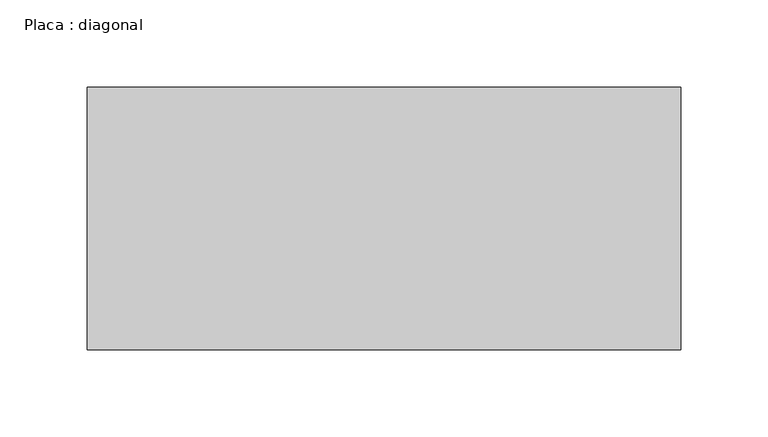
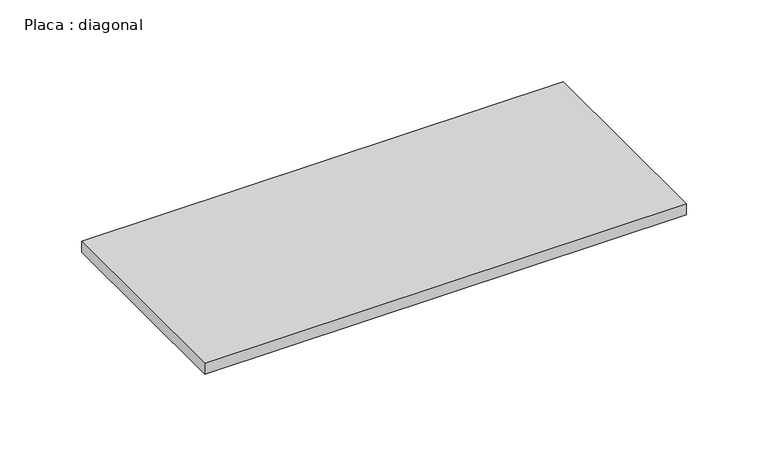
"""IFC4 building model written with IfcOpenShell, lengths in millimetres: beam geometry, Placa : diagonal."""

from ifc_helpers import new_model, si_unit, frame, origin, place, context, project, spatial, polyline, outline, extrude, source, transform, mapped, element, save


def placa_diagonal_668a1444(model_context):
    return source(origin(), model_context, "Body", "SweptSolid", [
        extrude(outline(polyline([(169.8505328, 75.0), (169.8505328, -75.0), (-169.6110753, -75.0), (-169.6110753, 75.0), (169.8505328, 75.0)])), frame((0.0, 0.0, -4.0), z_axis=(0.0, 0.0, 1.0), x_axis=(1.0, 0.0, 0.0)), (0.0, 0.0, 1.0), 8.0),
    ])


if __name__ == "__main__":
    model = new_model("IFC4")
    model_context = context("Model", 3, world=origin())
    ifc_project = project(units=[si_unit("LENGTHUNIT", "METRE", prefix="MILLI")], contexts=[model_context])
    site = spatial("IfcSite", under=ifc_project)
    building = spatial("IfcBuilding", under=site)
    placement = place(None, origin())
    placa_diagonal_shape = placa_diagonal_668a1444(model_context)
    element("IfcBeam", 1, ObjectType="Placa : diagonal", at=placement, inside=building, context=model_context, shape_type="MappedRepresentation", body=[
        mapped(placa_diagonal_shape, transform((0.0, 0.0, 0.0), x_axis=(1.0, 0.0, 0.0), y_axis=(0.0, 1.0, 0.0), z_axis=(0.0, 0.0, 1.0))),
    ])
    save(model, "model.ifc")

# Revit data of these elements
# Type "Placa : diagonal"
#   W = 0
#   Length [instance default] = 1.50 m
#   b = 0.15 m
#   d = 0.008 m
#   A = 0 m²
#   Structural Material [instance default] = Aço, 45-345
# Element 1 (IfcBeam, "Placa : diagonal")
#   Materials on its faces: "Aço, 45-345"
# Materials
#   "Aço, 45-345": class "Metal", colour RGB 247 247 247, transparency 0, Description = "Aço 345 MPa", Cost = 0
